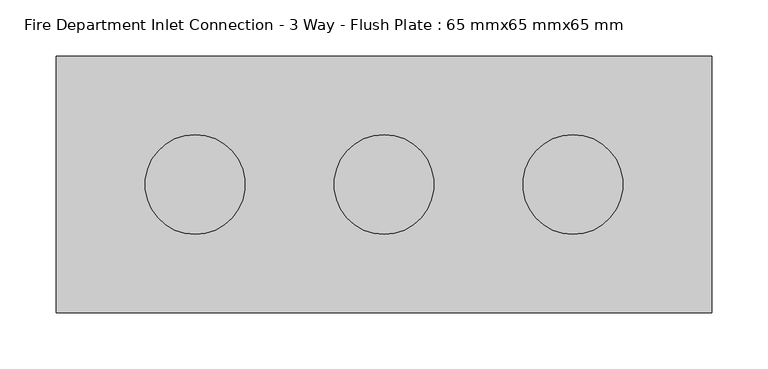
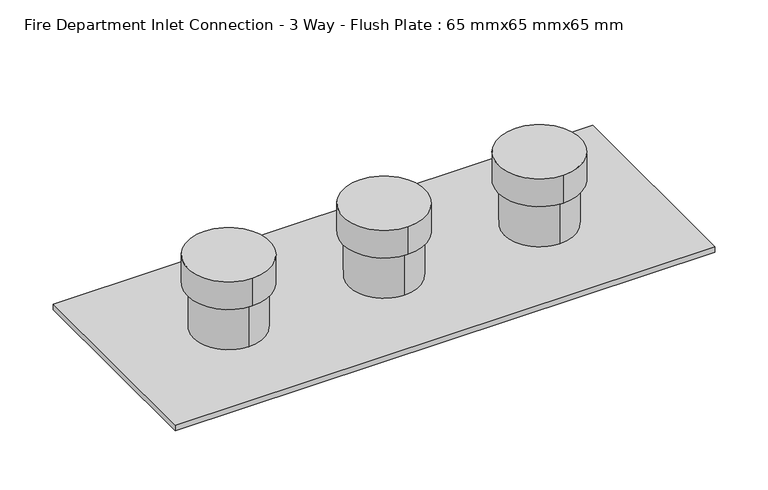
"""IFC4 building model written with IfcOpenShell, lengths in millimetres: proxy geometry, Fire Department Inlet Connection - 3 Way - Flush Plate : 65 mmx65 mmx65 mm."""

import ifcopenshell
import ifcopenshell.guid

model = None  # the IFC model being written
_history = None  # IfcOwnerHistory: only IFC2X3 demands one
_inside = {}  # id of a spatial element -> (the spatial element, [elements in it])
_under = {}  # id of a project, library or spatial element -> (it, [spatial elements below it])
_declared = {}  # id of a project -> (the project, [libraries it declares])
_typed = {}  # id of a type object -> (the type object, [elements of that type])
_made_of = {}  # id of a material, layer set ... -> (it, [elements and type objects made of it])


def new_model(schema):
    """Start an empty IFC model of exactly this schema.

    Asked for "IFC4X3", IfcOpenShell would pick the latest addendum, in which some entities
    have other attributes; the version numbers below select the first issue.
    IFC2X3 requires an IfcOwnerHistory on every rooted entity: one is made here for all.
    """
    global model, _history
    if schema == "IFC4X3":
        model = ifcopenshell.file(schema_version=(4, 3, 0, 0))
    else:
        model = ifcopenshell.file(schema=schema)
    _inside.clear()
    _under.clear()
    _declared.clear()
    _typed.clear()
    _made_of.clear()
    _history = None
    if model.schema == "IFC2X3":
        org = make("IfcOrganization", Name="unknown")
        user = make(
            "IfcPersonAndOrganization",
            ThePerson=make("IfcPerson", FamilyName="unknown"),
            TheOrganization=org,
        )
        app = make(
            "IfcApplication",
            ApplicationDeveloper=org,
            Version="unknown",
            ApplicationFullName="unknown",
            ApplicationIdentifier="unknown",
        )
        _history = make(
            "IfcOwnerHistory",
            OwningUser=user,
            OwningApplication=app,
            ChangeAction="ADDED",
            CreationDate=0,
        )
    return model


def make(cls, **values):
    """One entity of the class cls with the attributes given. An attribute that is None is left unset."""
    return model.create_entity(
        cls, **{name: value for name, value in values.items() if value is not None}
    )


def rooted(cls, **values):
    """An entity with a GlobalId (a new one), such as an element, a storey or a relation."""
    return make(cls, GlobalId=ifcopenshell.guid.new(), OwnerHistory=_history, **values)


def si_unit(unit_type, name, prefix=None):
    """IfcSIUnit, for example si_unit("LENGTHUNIT", "METRE", prefix="MILLI")."""
    return make("IfcSIUnit", UnitType=unit_type, Prefix=prefix, Name=name)


def assignment(units):
    """IfcUnitAssignment: the units of a project."""
    return None if units is None else make("IfcUnitAssignment", Units=units)


def point(xyz):
    """IfcCartesianPoint."""
    return None if xyz is None else make("IfcCartesianPoint", Coordinates=xyz)


def direction(xyz):
    """IfcDirection."""
    return None if xyz is None else make("IfcDirection", DirectionRatios=xyz)


def frame(location, z_axis=None, x_axis=None):
    """IfcAxis2Placement3D, a coordinate frame: its origin and axes. An axis left out is left unset."""
    return make(
        "IfcAxis2Placement3D",
        Location=point(location),
        Axis=direction(z_axis),
        RefDirection=direction(x_axis),
    )


def frame_2d(location, x_axis=None):
    """IfcAxis2Placement2D, a coordinate frame in the plane: its origin and x axis."""
    return make(
        "IfcAxis2Placement2D", Location=point(location), RefDirection=direction(x_axis)
    )


def origin():
    """The frame at (0, 0, 0) with its axes left unset."""
    return frame((0.0, 0.0, 0.0))


def origin_with_axes():
    """The frame at (0, 0, 0) with the z axis (0, 0, 1) and the x axis (1, 0, 0) written out."""
    return frame((0.0, 0.0, 0.0), z_axis=(0.0, 0.0, 1.0), x_axis=(1.0, 0.0, 0.0))


def origin_2d():
    """The frame at (0, 0) in the plane with its x axis left unset."""
    return frame_2d((0.0, 0.0))


def place(relative_to, where):
    """IfcLocalPlacement: puts the frame where relative to a parent placement (None: the world)."""
    return make(
        "IfcLocalPlacement", PlacementRelTo=relative_to, RelativePlacement=where
    )


def context(
    kind, dimensions, precision=None, world=None, true_north=None, identifier=None
):
    """IfcGeometricRepresentationContext, for example the 3D "Model" context."""
    return make(
        "IfcGeometricRepresentationContext",
        ContextIdentifier=identifier,
        ContextType=kind,
        CoordinateSpaceDimension=dimensions,
        Precision=precision,
        WorldCoordinateSystem=world,
        TrueNorth=true_north,
    )


def project(units=None, contexts=None):
    """IfcProject with its units and contexts."""
    return rooted(
        "IfcProject",
        Name="project",
        RepresentationContexts=contexts,
        UnitsInContext=assignment(units),
    )


def spatial(cls, under=None, at=None, **own):
    """A site, building, storey or space (cls), placed at a placement, below another one or the project."""
    s = rooted(cls, ObjectPlacement=at, **own)
    if under is not None:
        _under.setdefault(under.id(), (under, []))[1].append(s)
    return s


def polyline(points):
    """IfcPolyline through the points."""
    return make("IfcPolyline", Points=[point(p) for p in points])


def circle_curve(where, radius):
    """IfcCircle in the frame where."""
    return make("IfcCircle", Position=where, Radius=radius)


def trimmed(basis, trim1, trim2, sense, master):
    """IfcTrimmedCurve: the piece of a basis curve between two trims."""
    return make(
        "IfcTrimmedCurve",
        BasisCurve=basis,
        Trim1=trim1,
        Trim2=trim2,
        SenseAgreement=sense,
        MasterRepresentation=master,
    )


def segment(curve, same_sense, transition):
    """IfcCompositeCurveSegment."""
    return make(
        "IfcCompositeCurveSegment",
        Transition=transition,
        SameSense=same_sense,
        ParentCurve=curve,
    )


def composite_curve(segments, self_intersect=None):
    """IfcCompositeCurve: segments joined end to end."""
    return make("IfcCompositeCurve", Segments=segments, SelfIntersect=self_intersect)


def outline(outer, holes=None, kind="AREA"):
    """IfcArbitraryClosedProfileDef: a profile drawn as a closed curve; with holes, ...WithVoids."""
    if holes is None:
        return make("IfcArbitraryClosedProfileDef", ProfileType=kind, OuterCurve=outer)
    return make(
        "IfcArbitraryProfileDefWithVoids",
        ProfileType=kind,
        OuterCurve=outer,
        InnerCurves=holes,
    )


def extrude(swept, where, along, depth):
    """IfcExtrudedAreaSolid: the profile swept, set in the frame where, extruded along a direction by depth."""
    return make(
        "IfcExtrudedAreaSolid",
        SweptArea=swept,
        Position=where,
        ExtrudedDirection=direction(along),
        Depth=depth,
    )


def shape(context_of_items, identifier, shape_type, items):
    """IfcShapeRepresentation: the items that make up one representation, for example the "Body"."""
    return make(
        "IfcShapeRepresentation",
        ContextOfItems=context_of_items,
        RepresentationIdentifier=identifier,
        RepresentationType=shape_type,
        Items=items,
    )


def source(mapping_origin, context_of_items, identifier, shape_type, items):
    """IfcRepresentationMap: a shape defined once, which mapped items show again and again."""
    return make(
        "IfcRepresentationMap",
        MappingOrigin=mapping_origin,
        MappedRepresentation=shape(context_of_items, identifier, shape_type, items),
    )


def transform(
    local_origin,
    x_axis=None,
    y_axis=None,
    z_axis=None,
    scale=None,
    scale2=None,
    scale3=None,
    uniform=True,
):
    """IfcCartesianTransformationOperator3D, or its non-uniform kind. x_axis, y_axis, z_axis: its Axis1, 2, 3."""
    if uniform:
        return make(
            "IfcCartesianTransformationOperator3D",
            Axis1=direction(x_axis),
            Axis2=direction(y_axis),
            LocalOrigin=point(local_origin),
            Scale=scale,
            Axis3=direction(z_axis),
        )
    return make(
        "IfcCartesianTransformationOperator3DnonUniform",
        Axis1=direction(x_axis),
        Axis2=direction(y_axis),
        LocalOrigin=point(local_origin),
        Scale=scale,
        Axis3=direction(z_axis),
        Scale2=scale2,
        Scale3=scale3,
    )


def mapped(mapping_source, mapping_target):
    """IfcMappedItem: shows the shape of a source again, moved by a transform."""
    return make(
        "IfcMappedItem", MappingSource=mapping_source, MappingTarget=mapping_target
    )


def made_of(thing, what):
    """Note that an element or type object is made of a material, layer set ...; save() writes the relation."""
    if what is not None:
        _made_of.setdefault(what.id(), (what, []))[1].append(thing)
    return thing


def element(
    cls,
    number,
    at=None,
    inside=None,
    cuts=None,
    type_object=None,
    material=None,
    context=None,
    identifier="Body",
    shape_type=None,
    held_by="IfcProductDefinitionShape",
    body=None,
    shapes=None,
    **own,
):
    """One element of the class cls, such as IfcWall. Its Tag is "e" and its number.

    at: its placement. inside: the storey or other place that contains it. cuts: it is an
    opening in that element (IfcRelVoidsElement). A single representation is given by context,
    identifier, shape_type and body (its items); several are given by shapes. held_by: the class
    of the entity that holds the representations. save() writes the other relations.
    """
    e = rooted(cls, Tag="e%d" % number, ObjectPlacement=at, **own)
    if body is not None:
        shapes = [shape(context, identifier, shape_type, body)]
    if shapes is not None:
        e.Representation = make(held_by, Representations=shapes)
    if inside is not None:
        _inside.setdefault(inside.id(), (inside, []))[1].append(e)
    if cuts is not None:
        rooted(
            "IfcRelVoidsElement", RelatingBuildingElement=cuts, RelatedOpeningElement=e
        )
    if type_object is not None:
        _typed.setdefault(type_object.id(), (type_object, []))[1].append(e)
    return made_of(e, material)


def aggregate(whole, parts):
    """IfcRelAggregates: a whole, such as a stair, and the parts it consists of."""
    return rooted("IfcRelAggregates", RelatingObject=whole, RelatedObjects=parts)


def save(model, path):
    """Write the relations noted so far, then the file.

    IfcRelAggregates (storeys below a building ...), IfcRelContainedInSpatialStructure (elements
    in a storey), IfcRelDefinesByType, IfcRelAssociatesMaterial and IfcRelDeclares: one each for
    every whole, place, type object, material and project.
    """
    for whole, parts in _under.values():
        aggregate(whole, parts)
    for where, things in _inside.values():
        rooted(
            "IfcRelContainedInSpatialStructure",
            RelatedElements=things,
            RelatingStructure=where,
        )
    for kind, things in _typed.values():
        rooted("IfcRelDefinesByType", RelatedObjects=things, RelatingType=kind)
    for what, things in _made_of.values():
        rooted("IfcRelAssociatesMaterial", RelatedObjects=things, RelatingMaterial=what)
    for by, libraries in _declared.values():
        rooted("IfcRelDeclares", RelatingContext=by, RelatedDefinitions=libraries)
    model.write(path)


def plane_surface(at):
    """IfcPlane: the flat surface through the origin of the frame at, square to its z axis."""
    return make("IfcPlane", Position=at)


def cylinder_surface(at, radius):
    """IfcCylindricalSurface: all points at the distance radius from the z axis of the frame at."""
    return make("IfcCylindricalSurface", Position=at, Radius=radius)


def advanced_brep(points, edges, surfaces, faces):
    """IfcAdvancedBrep: a solid bounded by faces that lie on surfaces and meet in shared edges.

    An edge is (start, end): straight between two places in points (the first is 0);
    or (start, end, curve); or (start, end, curve, False) where it runs against its curve.
    A face is (place in surfaces, loops), or (place, loops, False) where it looks against
    its surface's normal. A loop lists edges by number (the first is 1), with a minus sign
    where the edge is run from its end to its start. The first loop is the outer one.
    """
    corners = [point(p) for p in points]
    vertices = [make("IfcVertexPoint", VertexGeometry=c) for c in corners]
    made = []
    for start, end, *more in edges:
        made.append(
            make(
                "IfcEdgeCurve",
                EdgeStart=vertices[start],
                EdgeEnd=vertices[end],
                EdgeGeometry=more[0] if more else make("IfcPolyline", Points=[corners[start], corners[end]]),
                SameSense=more[1] if len(more) > 1 else True,
            )
        )
    hull = []
    for where, loops, *sense in faces:
        bounds = []
        for j, loop in enumerate(loops):
            ring = [make("IfcOrientedEdge", EdgeElement=made[abs(k) - 1], Orientation=k > 0) for k in loop]
            bounds.append(
                make(
                    "IfcFaceOuterBound" if j == 0 else "IfcFaceBound",
                    Bound=make("IfcEdgeLoop", EdgeList=ring),
                    Orientation=True,
                )
            )
        hull.append(make("IfcAdvancedFace", Bounds=bounds, FaceSurface=surfaces[where], SameSense=sense[0] if sense else True))
    return make("IfcAdvancedBrep", Outer=make("IfcClosedShell", CfsFaces=hull))


def fire_department_inlet_connection_3_way_flush_plate_65_mmx65_f46b15d6(model_context):
    return source(origin(), model_context, "Body", "SolidModel", [
        extrude(outline(polyline([(292.1, 114.3), (292.1, -114.3), (-292.1, -114.3), (-292.1, 114.3), (292.1, 114.3)])), frame((0.0, 0.0, 6.35), z_axis=(0.0, 0.0, 1.0), x_axis=(1.0, 0.0, 0.0)), (0.0, 0.0, 1.0), 6.35),
        advanced_brep(
        [(168.275, 44.45, 95.25), (168.275, -44.45, 95.25), (168.275, 44.45, 63.5), (168.275, -44.45, 63.5), (168.275, 38.1, 63.5), (168.275, -38.1, 63.5), (168.275, 38.1, 12.7), (168.275, -38.1, 12.7)],
        [
            (0, 1, circle_curve(frame((168.275, 0.0, 95.25), z_axis=(0.0, 0.0, 1.0), x_axis=(0.0, -1.0, 0.0)), 44.45)),
            (1, 0, circle_curve(frame((168.275, 0.0, 95.25), z_axis=(0.0, 0.0, 1.0), x_axis=(0.0, -1.0, 0.0)), 44.45)),
            (2, 3, circle_curve(frame((168.275, 0.0, 63.5), z_axis=(0.0, 0.0, -1.0), x_axis=(0.0, -1.0, 0.0)), 44.45)),
            (3, 2, circle_curve(frame((168.275, 0.0, 63.5), z_axis=(0.0, 0.0, -1.0), x_axis=(0.0, -1.0, 0.0)), 44.45)),
            (4, 5, circle_curve(frame((168.275, 0.0, 63.5), z_axis=(0.0, 0.0, 1.0), x_axis=(0.0, -1.0, 0.0)), 38.1)),
            (5, 4, circle_curve(frame((168.275, 0.0, 63.5), z_axis=(0.0, 0.0, 1.0), x_axis=(0.0, -1.0, 0.0)), 38.1)),
            (0, 2),
            (3, 1),
            (6, 7, circle_curve(frame((168.275, 0.0, 12.7), z_axis=(0.0, 0.0, -1.0), x_axis=(0.0, -1.0, 0.0)), 38.1)),
            (7, 6, circle_curve(frame((168.275, 0.0, 12.7), z_axis=(0.0, 0.0, -1.0), x_axis=(0.0, -1.0, 0.0)), 38.1)),
            (7, 5),
            (4, 6),
        ],
        [
            plane_surface(frame((168.275, -44.45, 95.25), z_axis=(0.0, 0.0, 1.0), x_axis=(1.0, 0.0, 0.0))),
            plane_surface(frame((168.275, -44.45, 63.5), z_axis=(0.0, 0.0, -1.0), x_axis=(-1.0, 0.0, 0.0))),
            cylinder_surface(frame((168.275, 0.0, 63.5), z_axis=(0.0, 0.0, 1.0), x_axis=(0.0, -1.0, 0.0)), 44.45),
            plane_surface(frame((168.275, -38.1, 12.7), z_axis=(0.0, 0.0, -1.0), x_axis=(-1.0, 0.0, 0.0))),
            cylinder_surface(frame((168.275, 0.0, 12.7), z_axis=(0.0, 0.0, 1.0), x_axis=(0.0, -1.0, 0.0)), 38.1),
        ],
        [
            (0, [[1, 2]]),
            (1, [[3, 4], [5, 6]]),
            (2, [[-1, 7, -4, 8]]),
            (2, [[-2, -8, -3, -7]]),
            (3, [[9, 10]]),
            (4, [[-10, 11, -5, 12]]),
            (4, [[-9, -12, -6, -11]]),
        ],
    ),
        advanced_brep(
        [(0.0, 44.45, 95.25), (0.0, -44.45, 95.25), (0.0, 44.45, 63.5), (0.0, -44.45, 63.5), (0.0, 38.1, 63.5), (0.0, -38.1, 63.5), (0.0, 38.1, 12.7), (0.0, -38.1, 12.7)],
        [
            (0, 1, circle_curve(frame((0.0, 0.0, 95.25), z_axis=(0.0, 0.0, 1.0), x_axis=(0.0, -1.0, 0.0)), 44.45)),
            (1, 0, circle_curve(frame((0.0, 0.0, 95.25), z_axis=(0.0, 0.0, 1.0), x_axis=(0.0, -1.0, 0.0)), 44.45)),
            (2, 3, circle_curve(frame((0.0, 0.0, 63.5), z_axis=(0.0, 0.0, -1.0), x_axis=(0.0, -1.0, 0.0)), 44.45)),
            (3, 2, circle_curve(frame((0.0, 0.0, 63.5), z_axis=(0.0, 0.0, -1.0), x_axis=(0.0, -1.0, 0.0)), 44.45)),
            (4, 5, circle_curve(frame((0.0, 0.0, 63.5), z_axis=(0.0, 0.0, 1.0), x_axis=(0.0, -1.0, 0.0)), 38.1)),
            (5, 4, circle_curve(frame((0.0, 0.0, 63.5), z_axis=(0.0, 0.0, 1.0), x_axis=(0.0, -1.0, 0.0)), 38.1)),
            (0, 2),
            (3, 1),
            (6, 7, circle_curve(frame((0.0, 0.0, 12.7), z_axis=(0.0, 0.0, -1.0), x_axis=(0.0, -1.0, 0.0)), 38.1)),
            (7, 6, circle_curve(frame((0.0, 0.0, 12.7), z_axis=(0.0, 0.0, -1.0), x_axis=(0.0, -1.0, 0.0)), 38.1)),
            (7, 5),
            (4, 6),
        ],
        [
            plane_surface(frame((168.275, -44.45, 95.25), z_axis=(0.0, 0.0, 1.0), x_axis=(1.0, 0.0, 0.0))),
            plane_surface(frame((168.275, -44.45, 63.5), z_axis=(0.0, 0.0, -1.0), x_axis=(-1.0, 0.0, 0.0))),
            cylinder_surface(frame((0.0, 0.0, 0.0), z_axis=(0.0, 0.0, 1.0), x_axis=(0.0, -1.0, 0.0)), 44.45),
            plane_surface(frame((168.275, -38.1, 12.7), z_axis=(0.0, 0.0, -1.0), x_axis=(-1.0, 0.0, 0.0))),
            cylinder_surface(frame((0.0, 0.0, 0.0), z_axis=(0.0, 0.0, 1.0), x_axis=(0.0, -1.0, 0.0)), 38.1),
        ],
        [
            (0, [[1, 2]]),
            (1, [[3, 4], [5, 6]]),
            (2, [[-1, 7, -4, 8]]),
            (2, [[-2, -8, -3, -7]]),
            (3, [[9, 10]]),
            (4, [[-10, 11, -5, 12]]),
            (4, [[-9, -12, -6, -11]]),
        ],
    ),
        advanced_brep(
        [(-168.275, 44.45, 95.25), (-168.275, -44.45, 95.25), (-168.275, 44.45, 63.5), (-168.275, -44.45, 63.5), (-168.275, 38.1, 63.5), (-168.275, -38.1, 63.5), (-168.275, 38.1, 12.7), (-168.275, -38.1, 12.7)],
        [
            (0, 1, circle_curve(frame((-168.275, 0.0, 95.25), z_axis=(0.0, 0.0, 1.0), x_axis=(0.0, -1.0, 0.0)), 44.45)),
            (1, 0, circle_curve(frame((-168.275, 0.0, 95.25), z_axis=(0.0, 0.0, 1.0), x_axis=(0.0, -1.0, 0.0)), 44.45)),
            (2, 3, circle_curve(frame((-168.275, 0.0, 63.5), z_axis=(0.0, 0.0, -1.0), x_axis=(0.0, -1.0, 0.0)), 44.45)),
            (3, 2, circle_curve(frame((-168.275, 0.0, 63.5), z_axis=(0.0, 0.0, -1.0), x_axis=(0.0, -1.0, 0.0)), 44.45)),
            (4, 5, circle_curve(frame((-168.275, 0.0, 63.5), z_axis=(0.0, 0.0, 1.0), x_axis=(0.0, -1.0, 0.0)), 38.1)),
            (5, 4, circle_curve(frame((-168.275, 0.0, 63.5), z_axis=(0.0, 0.0, 1.0), x_axis=(0.0, -1.0, 0.0)), 38.1)),
            (0, 2),
            (3, 1),
            (6, 7, circle_curve(frame((-168.275, 0.0, 12.7), z_axis=(0.0, 0.0, -1.0), x_axis=(0.0, -1.0, 0.0)), 38.1)),
            (7, 6, circle_curve(frame((-168.275, 0.0, 12.7), z_axis=(0.0, 0.0, -1.0), x_axis=(0.0, -1.0, 0.0)), 38.1)),
            (7, 5),
            (4, 6),
        ],
        [
            plane_surface(frame((168.275, -44.45, 95.25), z_axis=(0.0, 0.0, 1.0), x_axis=(1.0, 0.0, 0.0))),
            plane_surface(frame((168.275, -44.45, 63.5), z_axis=(0.0, 0.0, -1.0), x_axis=(-1.0, 0.0, 0.0))),
            cylinder_surface(frame((-168.275, 0.0, 0.0), z_axis=(0.0, 0.0, 1.0), x_axis=(0.0, -1.0, 0.0)), 44.45),
            plane_surface(frame((168.275, -38.1, 12.7), z_axis=(0.0, 0.0, -1.0), x_axis=(-1.0, 0.0, 0.0))),
            cylinder_surface(frame((-168.275, 0.0, 0.0), z_axis=(0.0, 0.0, 1.0), x_axis=(0.0, -1.0, 0.0)), 38.1),
        ],
        [
            (0, [[1, 2]]),
            (1, [[3, 4], [5, 6]]),
            (2, [[-1, 7, -4, 8]]),
            (2, [[-2, -8, -3, -7]]),
            (3, [[9, 10]]),
            (4, [[-10, 11, -5, 12]]),
            (4, [[-9, -12, -6, -11]]),
        ],
    ),
        extrude(outline(composite_curve([segment(trimmed(circle_curve(frame_2d((168.275, 0.0)), 50.8), [point((168.275, 50.8))], [point((168.275, -50.8))], False, "CARTESIAN"), True, "CONTINUOUS"), segment(trimmed(circle_curve(frame_2d((168.275, 0.0)), 50.8), [point((168.275, -50.8))], [point((168.275, 50.8))], False, "CARTESIAN"), True, "CONTINUOUS")], self_intersect=False)), origin_with_axes(), (0.0, 0.0, 1.0), 6.35),
        extrude(outline(composite_curve([segment(trimmed(circle_curve(origin_2d(), 50.8), [point((0.0, 50.8))], [point((0.0, -50.8))], False, "CARTESIAN"), True, "CONTINUOUS"), segment(trimmed(circle_curve(origin_2d(), 50.8), [point((0.0, -50.8))], [point((0.0, 50.8))], False, "CARTESIAN"), True, "CONTINUOUS")], self_intersect=False)), origin_with_axes(), (0.0, 0.0, 1.0), 6.35),
        extrude(outline(composite_curve([segment(trimmed(circle_curve(frame_2d((-168.275, 0.0)), 50.8), [point((-168.275, 50.8))], [point((-168.275, -50.8))], False, "CARTESIAN"), True, "CONTINUOUS"), segment(trimmed(circle_curve(frame_2d((-168.275, 0.0)), 50.8), [point((-168.275, -50.8))], [point((-168.275, 50.8))], False, "CARTESIAN"), True, "CONTINUOUS")], self_intersect=False)), origin_with_axes(), (0.0, 0.0, 1.0), 6.35),
    ])


if __name__ == "__main__":
    model = new_model("IFC4")
    model_context = context("Model", 3, world=origin())
    ifc_project = project(units=[si_unit("LENGTHUNIT", "METRE", prefix="MILLI")], contexts=[model_context])
    site = spatial("IfcSite", under=ifc_project)
    building = spatial("IfcBuilding", under=site)
    placement = place(None, origin())
    fire_department_inlet_connection_3_way_flush_plate_65_mmx65_shape = fire_department_inlet_connection_3_way_flush_plate_65_mmx65_f46b15d6(model_context)
    element("IfcBuildingElementProxy", 1, Name="Fire Department Inlet Connection - 3 Way - Flush Plate : 65 mmx65 mmx65 mm", ObjectType="Fire Department Inlet Connection - 3 Way - Flush Plate : 65 mmx65 mmx65 mm", at=placement, inside=building, context=model_context, shape_type="MappedRepresentation", body=[
        mapped(fire_department_inlet_connection_3_way_flush_plate_65_mmx65_shape, transform((0.0, 0.0, 0.0), x_axis=(1.0, 0.0, 0.0), y_axis=(0.0, 1.0, 0.0), z_axis=(0.0, 0.0, 1.0))),
    ])
    save(model, "model.ifc")

# Revit data of these elements
# Project information
#   Sheet x = "1"
#   Sheet Total = "4"
#   COBie.CreatedBy = "info@mma.ie"
#   COBie.CreatedOn = "2017-07-04T11:33:08"
#   COBie.Facility.Category = "11-16 27 14 : Mixed-Gender Dormitory"
#   COBie.Facility.ProjectName = "East Dormitory"
#   COBie.Facility.SiteName = "East Healey Street, Champaign, Illinois, USA"
#   COBie.Facility.LinearUnits = "Millimeters"
#   COBie.Facility.AreaUnits = "Square Meters"
#   COBie.Facility.VolumeUnits = "Cubic Meters"
#   COBie.Facility.CurrencyUnit = "None"
#   COBie.Facility.AreaMeasurement = "Revit Default Area Calculation Method"
#   COBie.Facility.Description = "Two Storey Luxury Dormitory"
#   COBie.Facility.ProjectDescription = "One of Four Dormitories on the E.Healey Site"
#   COBie.Facility.SiteDescription = "Four Dormitories Project Site"
#   COBie.Facility.Phase = "60% Design Submission"
#   Classification.Facility.Description = "Mixed-Gender Dormitory"
#   Classification.Facility.Number = "11-16 27 14"
#   Project Issue Date = "Issue Date"
#   Project Status = "Final Issue"
#   Client Name = "Prairie Sky Consulting"
#   Project Address = "East Healey Street, \nChampaign, \nIllinois, \nUSA"
#   Project Name = "Four Dormitory Complex"
#   Project Number = "East Dormitory"
# Type "Fire Department Inlet Connection - 3 Way - Flush Plate : 65 mmx65 mmx65 mm"
#   Type Mark = "Fire Department Inlet Connection - 3 Way - Flush Plate"
#   COBie.Type.CreatedBy = "info@mma.ie"
#   COBie.Type.CreatedOn = "2017-07-04T11:33:08"
#   COBie.Type.Name = "Fire Department Inlet Connection - 3 Way - Flush Plate"
#   COBie.Type.Category = "23-29 25 15 : Fire Hose Equipment"
#   COBie.Type.Description = "Fire Department Inlet Connection - 3 Way - Flush Plate_65 mmx65 mmx65 mm"
#   COBie.Type.AssetType = "Fixed"
#   COBie.Type.Manufacturer = ""
#   COBie.Type.ModelNumber = ""
#   COBie.Type.ModelReference = "21 11 19.A"
#   Classification.OmniClass.23.Number = "23-29 25 15"
#   Classification.OmniClass.23.Description = "Fire Hose Equipment"
#   Keynote = "21 11 19.A"
#   F.I.-Material = "Polished Brass Plate"
#   F.I.-Inlet = ""
#   F.I. No. of Inlets = "3"
#   COBie.Type.ReplacementCost = 0
#   Nominal Radius = 32.5 mm
#   Nominal Diameter = 65 mm
#   F.I. Inlet = 88.9 mm
#   Default Elevation = 700 mm
#   COBie.Type = yes
#   Inlet Connection Plate Material = Polished Brass
# Element 1 (IfcBuildingElementProxy, "Fire Department Inlet Connection - 3 Way - Flush Plate : 65 mmx65 mmx65 mm")
#   Materials on its faces: "Polished Brass"
# Materials
#   "Polished Brass": class "Plastic", colour RGB 120 120 120, transparency 0, Description = "Acrylonitrile butadiene styrene", Cost = 0
